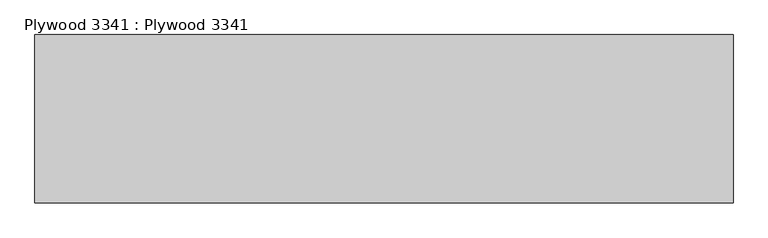
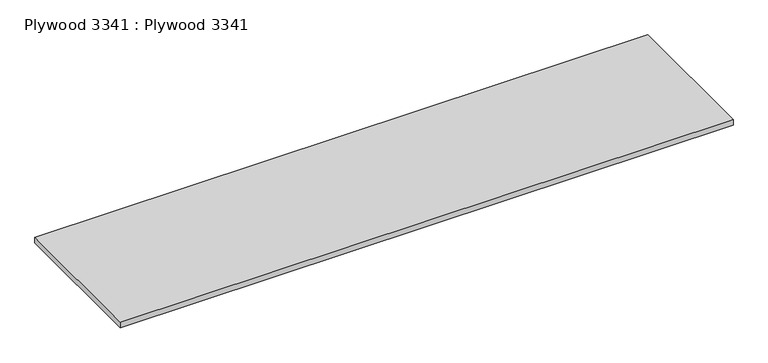
"""IFC4 building model written with IfcOpenShell, lengths in millimetres: proxy geometry, Plywood 3341 : Plywood 3341."""

from ifc_helpers import new_model, si_unit, frame, origin, place, context, project, spatial, polyline, outline, extrude, source, transform, mapped, element, save


def plywood_3341_plywood_3341_3baffb16(model_context):
    return source(origin(), model_context, "Body", "SweptSolid", [
        extrude(outline(polyline([(3694.2883192, 9750.662737), (3694.2883192, 10233.2619974), (5694.2883192, 10233.2619974), (5694.2883192, 9750.662737), (3694.2883192, 9750.662737)])), frame((0.0, 0.0, 39738.0485313), z_axis=(0.0, 0.0, 1.0), x_axis=(1.0, 0.0, 0.0)), (0.0, 0.0, 1.0), 19.049125),
    ])


if __name__ == "__main__":
    model = new_model("IFC4")
    model_context = context("Model", 3, world=origin())
    ifc_project = project(units=[si_unit("LENGTHUNIT", "METRE", prefix="MILLI")], contexts=[model_context])
    site = spatial("IfcSite", under=ifc_project)
    building = spatial("IfcBuilding", under=site)
    placement = place(None, origin())
    plywood_3341_plywood_3341_shape = plywood_3341_plywood_3341_3baffb16(model_context)
    element("IfcBuildingElementProxy", 1, Name="Plywood 3341 : Plywood 3341", ObjectType="Plywood 3341 : Plywood 3341", at=placement, inside=building, context=model_context, shape_type="MappedRepresentation", body=[
        mapped(plywood_3341_plywood_3341_shape, transform((0.0, 0.0, 0.0), x_axis=(1.0, 0.0, 0.0), y_axis=(0.0, 1.0, 0.0), z_axis=(0.0, 0.0, 1.0))),
    ])
    save(model, "model.ifc")

# Revit data of these elements
# Type "Plywood 3341 : Plywood 3341"
#   NameOverride = "Plywood"
# Element 1 (IfcBuildingElementProxy, "Plywood 3341 : Plywood 3341")
#   Materials on its faces: "CDX PLYWOOD -  SEE STRUCTURAL DWGS"
# Materials
#   "CDX PLYWOOD -  SEE STRUCTURAL DWGS": class "Unassigned", colour RGB 177 130 114, transparency 0, Cost = 0
